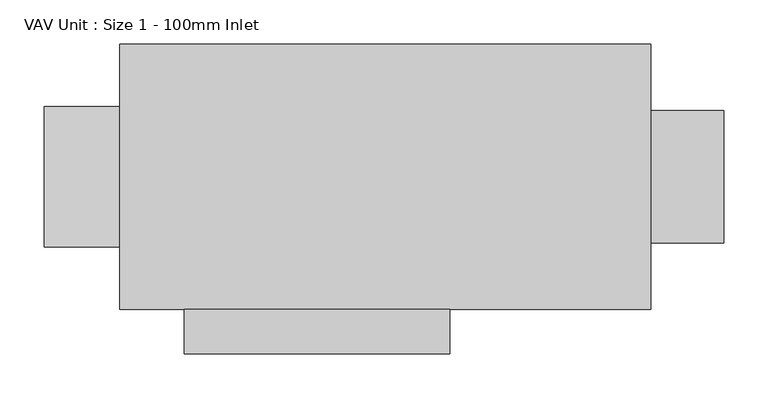
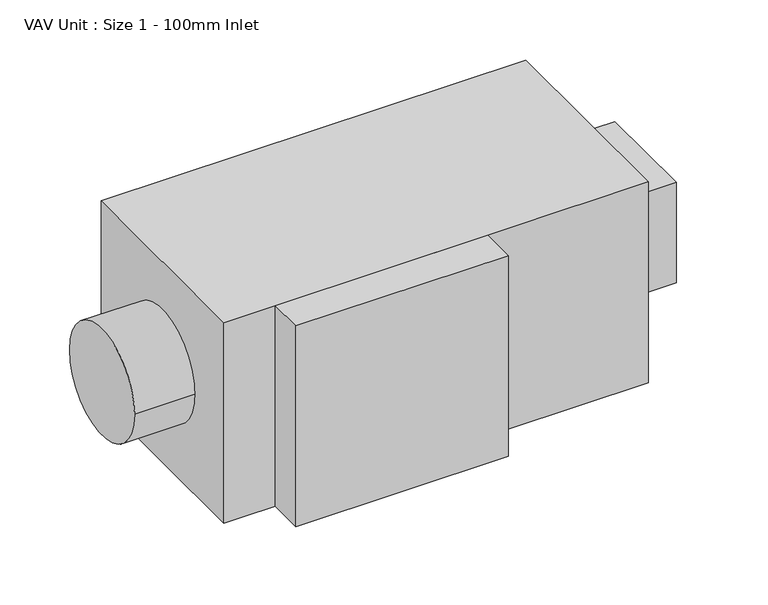
"""IFC4 building model written with IfcOpenShell, lengths in millimetres: proxy geometry, VAV Unit : Size 1 - 100mm Inlet."""

from ifc_helpers import new_model, si_unit, point, frame, origin, origin_2d, place, context, project, spatial, polyline, circle_curve, trimmed, segment, composite_curve, outline, extrude, source, transform, mapped, element, save


def vav_unit_size_1_100mm_inlet_84ca79ad(model_context):
    return source(origin(), model_context, "Body", "SweptSolid", [
        extrude(outline(polyline([(382.4821717, -75.0), (300.0, -75.0), (300.0, 75.0), (382.4821717, 75.0), (382.4821717, -75.0)])), frame((0.0, 0.0, -75.0), z_axis=(0.0, 0.0, 1.0), x_axis=(1.0, 0.0, 0.0)), (0.0, 0.0, 1.0), 150.0),
        extrude(outline(polyline([(73.0, -150.0), (73.0, -200.0), (-227.0, -200.0), (-227.0, -150.0), (73.0, -150.0)])), frame((0.0, 0.0, -150.0), z_axis=(0.0, 0.0, 1.0), x_axis=(1.0, 0.0, 0.0)), (0.0, 0.0, 1.0), 300.0),
        extrude(outline(composite_curve([segment(trimmed(circle_curve(origin_2d(), 79.5), [point((79.5, 0.0))], [point((-79.5, 0.0))], False, "CARTESIAN"), True, "CONTINUOUS"), segment(trimmed(circle_curve(origin_2d(), 79.5), [point((-79.5, 0.0))], [point((79.5, 0.0))], False, "CARTESIAN"), True, "CONTINUOUS")], self_intersect=False)), frame((-385.0, 0.0, 0.0), z_axis=(1.0, 0.0, 0.0), x_axis=(0.0, 1.0, 0.0)), (0.0, 0.0, 1.0), 85.0),
        extrude(outline(polyline([(300.0, -150.0), (-300.0, -150.0), (-300.0, 150.0), (300.0, 150.0), (300.0, -150.0)])), frame((0.0, 0.0, -150.0), z_axis=(0.0, 0.0, 1.0), x_axis=(1.0, 0.0, 0.0)), (0.0, 0.0, 1.0), 300.0),
    ])


if __name__ == "__main__":
    model = new_model("IFC4")
    model_context = context("Model", 3, world=origin())
    ifc_project = project(units=[si_unit("LENGTHUNIT", "METRE", prefix="MILLI")], contexts=[model_context])
    site = spatial("IfcSite", under=ifc_project)
    building = spatial("IfcBuilding", under=site)
    placement = place(None, origin())
    vav_unit_size_1_100mm_inlet_shape = vav_unit_size_1_100mm_inlet_84ca79ad(model_context)
    element("IfcBuildingElementProxy", 1, Name="VAV Unit : Size 1 - 100mm Inlet", ObjectType="VAV Unit : Size 1 - 100mm Inlet", at=placement, inside=building, context=model_context, shape_type="MappedRepresentation", body=[
        mapped(vav_unit_size_1_100mm_inlet_shape, transform((0.0, 0.0, 0.0), x_axis=(1.0, 0.0, 0.0), y_axis=(0.0, 1.0, 0.0), z_axis=(0.0, 0.0, 1.0))),
    ])
    save(model, "model.ifc")

# Revit data of these elements
# Type "VAV Unit : Size 1 - 100mm Inlet"
#   Type Mark = "VAV Unit"
#   COBie.Type.CreatedBy = "info@mma.ie"
#   COBie.Type.CreatedOn = "2017-07-21T10:57:54"
#   COBie.Type.Name = "VAV Unit"
#   COBie.Type.Category = "23-33 41 17 13 : Variable Air Volume Terminal Units"
#   COBie.Type.Description = "VAV Unit_Size 1 - 100mm Inlet"
#   COBie.Type.AssetType = "Fixed"
#   COBie.Type.Manufacturer = ""
#   COBie.Type.ModelNumber = ""
#   COBie.Type.ModelReference = ""
#   Classification.OmniClass.23.Number = "23-33 41 17 13"
#   Classification.OmniClass.23.Description = "Variable Air Volume Terminal Units"
#   Keynote = "23 36 16.A"
#   COBie.Type.ReplacementCost = 0
#   Width2 = 150 mm
#   Voltage = 230 V
#   UnitWidth = 600 mm
#   UnitHeight = 300 mm
#   UnitDepth = 300 mm
#   Unit Weight = 300 mm
#   Unit Lenght = 600 mm
#   Unit Height = 300 mm
#   SupplyConnectorWidth = 150 mm
#   SupplyConnectorVerticalOffset = 54 mm
#   SupplyConnectorLength = 15 mm
#   SupplyConnectorHorizontalOffset = 90 mm
#   SupplyConnectorDepth = 150 mm
#   SupplyAirConnectorCenterOffset = 165 mm
#   Static Pressure [instance default] = 0.0401865 in-wg
#   PrimaryToSupplyRatio [instance default] = 0.2
#   PrimaryAirOffset = 150 mm
#   PrimaryAirFlow [instance default] = 100.011 CFM
#   PrimaryAirConnectorVerticalOffset = 150 mm
#   PrimaryAirConnectorRadius = 79.5 mm
#   PrimaryAirConnectorLength = 85 mm
#   PrimaryAirConnectorDiameter = 159 mm
#   PrimaryAirConnectorCenterOffset = 150 mm
#   InducedAirInletWidth = 400 mm
#   InducedAirInletDepth = 350 mm
#   InducedAirConnectorHorizontalOffset = 25 mm
#   InducedAirConnectorCenterOffset = 225 mm
#   Height2 = 150 mm
#   ElectricalConnectionBoxWidth = 300 mm
#   ElectricalConnectionBoxOffset = 73 mm
#   ElectricalConnectionBoxHeight = 50 mm
#   ElectricalConnectionBoxDepth = 300 mm
#   Apparent Load = 181 VA
#   Air Flow [instance default] = 500.056 CFM
#   COBie.Type = yes
#   SupplyAirConnectorIndex = 2
#   PrimaryAirConnectorIndex = 1
#   Number of Poles = 1
#   InducedAirConnectorIndex = 3
#   VAV Material = none
#   Load Classification = Cooling
#   Default Elevation = 0
#   Assembly Code = ""
# Element 1 (IfcBuildingElementProxy, "VAV Unit : Size 1 - 100mm Inlet")
#   Static Pressure = 0.1 in-wg
#   PrimaryAirFlow = 14.8322 CFM
#   Air Flow = 74.1608 CFM
